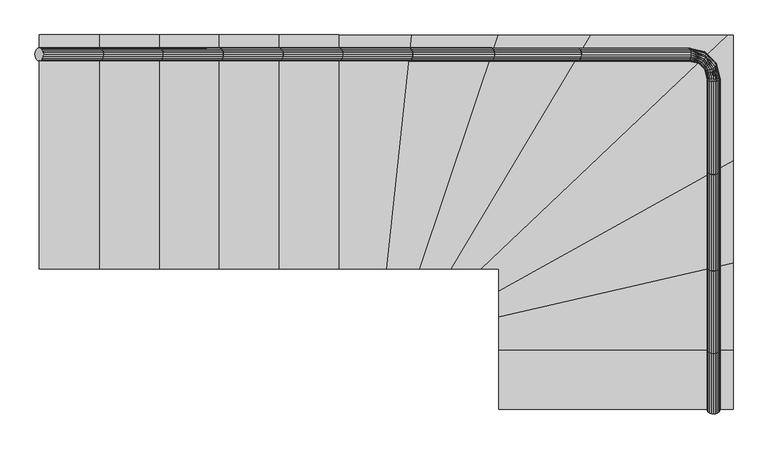
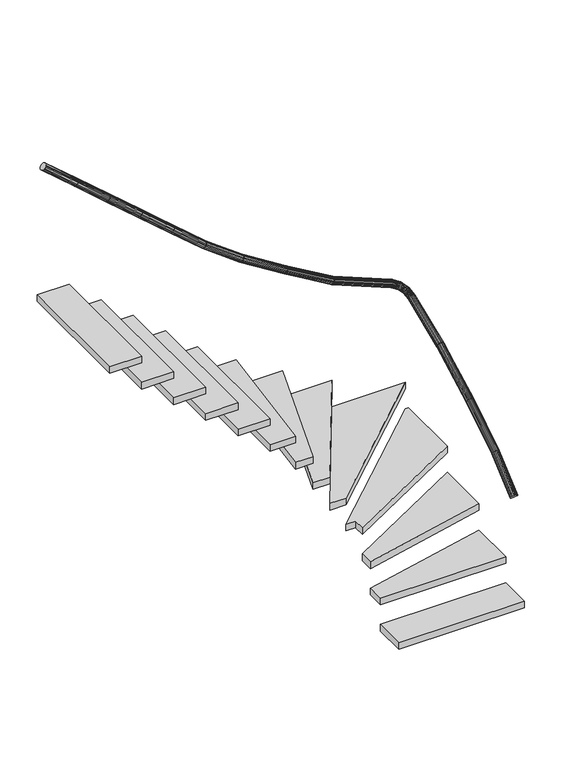
"""IFC4 building model written with IfcOpenShell, lengths in millimetres: stair geometry, 0_3d."""

from ifc_helpers import new_model, si_unit, frame, origin, origin_with_axes, place, context, project, spatial, polyline, outline, extrude, faceted_brep, source, transform, mapped, element, save


def stair_b834b6f4(model_context):
    return source(origin(), model_context, "Body", "SolidModel", [
        faceted_brep([(1747.6382113, 1405.678272, 2054.1646194), (1751.801684, 1406.9018591, 2060.987808), (1755.9651567, 1405.678272, 2067.8109967), (1759.7210797, 1402.127284, 2073.966284), (1762.701797, 1396.5964904, 2078.8511477), (1764.6155354, 1389.627284, 2081.9874233), (1765.2749647, 1381.9018591, 2083.0681102), (1764.6155354, 1374.1764343, 2081.9874233), (1762.701797, 1367.2072278, 2078.8511477), (1759.7210797, 1361.6764343, 2073.966284), (1755.9651567, 1358.1254462, 2067.8109967), (1751.801684, 1356.9018591, 2060.987808), (1747.6382113, 1358.1254462, 2054.1646194), (1743.8822884, 1361.6764343, 2048.009332), (1740.901571, 1367.2072278, 2043.1244683), (1738.9878327, 1374.1764343, 2039.9881928), (1738.3284034, 1381.9018591, 2038.9075058), (1738.9878327, 1389.627284, 2039.9881928), (1740.901571, 1396.5964904, 2043.1244683), (1743.8822884, 1402.127284, 2048.009332), (1441.1651504, 1405.678272, 2266.1670868), (1436.659926, 1406.9018591, 2259.5592366), (1432.1547015, 1405.678272, 2252.9513864), (1428.0904799, 1402.127284, 2246.9903587), (1424.8650953, 1396.5964904, 2242.2596602), (1422.7942709, 1389.627284, 2239.2223649), (1422.0807134, 1381.9018591, 2238.1757842), (1422.7942709, 1374.1764343, 2239.2223649), (1424.8650953, 1367.2072278, 2242.2596602), (1428.0904799, 1361.6764343, 2246.9903587), (1432.1547015, 1358.1254462, 2252.9513864), (1436.659926, 1356.9018591, 2259.5592366), (1441.1651504, 1358.1254462, 2266.1670868), (1445.2293721, 1361.6764343, 2272.1281145), (1448.4547567, 1367.2072278, 2276.858813), (1450.5255811, 1374.1764343, 2279.8961083), (1451.2391385, 1381.9018591, 2280.942689), (1450.5255811, 1389.627284, 2279.8961083), (1448.4547567, 1396.5964904, 2276.858813), (1445.2293721, 1402.127284, 2272.1281145)], [[[0, 1, 2, 3, 4, 5, 6, 7, 8, 9, 10, 11, 12, 13, 14, 15, 16, 17, 18, 19]], [[20, 21, 22, 23, 24, 25, 26, 27, 28, 29, 30, 31, 32, 33, 34, 35, 36, 37, 38, 39]], [[2, 1, 21, 20]], [[3, 2, 20, 39]], [[4, 3, 39, 38]], [[5, 4, 38, 37]], [[6, 5, 37, 36]], [[7, 6, 36, 35]], [[8, 7, 35, 34]], [[9, 8, 34, 33]], [[10, 9, 33, 32]], [[11, 10, 32, 31]], [[12, 11, 31, 30]], [[13, 12, 30, 29]], [[14, 13, 29, 28]], [[15, 14, 28, 27]], [[16, 15, 27, 26]], [[17, 16, 26, 25]], [[18, 17, 25, 24]], [[19, 18, 24, 23]], [[0, 19, 23, 22]], [[1, 0, 22, 21]]]),
        faceted_brep([(2630.2801086, 566.7337566, 1259.7925307), (2631.5036957, 562.7078511, 1266.7020937), (2630.2801086, 558.6819455, 1273.6116568), (2626.7291206, 555.0501237, 1279.8448636), (2621.198327, 552.1678935, 1284.7915646), (2614.2291206, 550.3173878, 1287.9675421), (2606.5036957, 549.679747, 1289.0619094), (2598.7782709, 550.3173878, 1287.9675421), (2591.8090644, 552.1678935, 1284.7915646), (2586.2782709, 555.0501237, 1279.8448636), (2582.7272828, 558.6819455, 1273.6116568), (2581.5036957, 562.7078511, 1266.7020937), (2582.7272828, 566.7337566, 1259.7925307), (2586.2782709, 570.3655785, 1253.5593239), (2591.8090644, 573.2478087, 1248.6126229), (2598.7782709, 575.0983143, 1245.4366454), (2606.5036957, 575.7359551, 1244.3422781), (2614.2291206, 575.0983143, 1245.4366454), (2621.198327, 573.2478087, 1248.6126229), (2626.7291206, 570.3655785, 1253.5593239), (2630.2801086, 928.1440687, 1472.4992177), (2631.5036957, 931.5827131, 1465.2735223), (2630.2801086, 935.0213576, 1458.0478269), (2626.7291206, 938.1234035, 1451.529433), (2621.198327, 940.5852011, 1446.3564062), (2614.2291206, 942.1657724, 1443.0351186), (2606.5036957, 942.7104002, 1441.8906809), (2598.7782709, 942.1657724, 1443.0351186), (2591.8090644, 940.5852011, 1446.3564062), (2586.2782709, 938.1234035, 1451.529433), (2582.7272828, 935.0213576, 1458.0478269), (2581.5036957, 931.5827131, 1465.2735223), (2582.7272828, 928.1440687, 1472.4992177), (2586.2782709, 925.0420228, 1479.0176117), (2591.8090644, 922.5802252, 1484.1906384), (2598.7782709, 920.9996538, 1487.511926), (2606.5036957, 920.4550261, 1488.6563638), (2614.2291206, 920.9996538, 1487.511926), (2621.198327, 922.5802252, 1484.1906384), (2626.7291206, 925.0420228, 1479.0176117)], [[[0, 1, 2, 3, 4, 5, 6, 7, 8, 9, 10, 11, 12, 13, 14, 15, 16, 17, 18, 19]], [[20, 21, 22, 23, 24, 25, 26, 27, 28, 29, 30, 31, 32, 33, 34, 35, 36, 37, 38, 39]], [[2, 1, 21, 20]], [[3, 2, 20, 39]], [[4, 3, 39, 38]], [[5, 4, 38, 37]], [[6, 5, 37, 36]], [[7, 6, 36, 35]], [[8, 7, 35, 34]], [[9, 8, 34, 33]], [[10, 9, 33, 32]], [[11, 10, 32, 31]], [[12, 11, 31, 30]], [[13, 12, 30, 29]], [[14, 13, 29, 28]], [[15, 14, 28, 27]], [[16, 15, 27, 26]], [[17, 16, 26, 25]], [[18, 17, 25, 24]], [[19, 18, 24, 23]], [[0, 19, 23, 22]], [[1, 0, 22, 21]]]),
        extrude(outline(polyline([(1781.5036957, 246.9018591), (1781.5036957, 373.9346688), (2681.5036957, 579.8690495), (2681.5036957, 246.9018591), (1781.5036957, 246.9018591)])), frame((0.0, 0.0, 198.5714286), z_axis=(0.0, 0.0, 1.0), x_axis=(1.0, 0.0, 0.0)), (0.0, 0.0, 1.0), 50.0),
        extrude(outline(polyline([(706.9018591, 556.9018591), (476.9018591, 556.9018591), (476.9018591, 1456.9018591), (706.9018591, 1456.9018591), (706.9018591, 556.9018591)])), frame((0.0, 0.0, 1985.7142857), z_axis=(0.0, 0.0, 1.0), x_axis=(1.0, 0.0, 0.0)), (0.0, 0.0, 1.0), 50.0),
        extrude(outline(polyline([(1781.5036957, 473.824936), (1781.5036957, 556.9018591), (1711.5036957, 556.9018591), (2658.8332796, 1456.9018591), (2681.5036957, 1456.9018591), (2681.5036957, 973.1970565), (1781.5036957, 473.824936)])), frame((0.0, 0.0, 595.7142857), z_axis=(0.0, 0.0, 1.0), x_axis=(1.0, 0.0, 0.0)), (0.0, 0.0, 1.0), 50.0),
        extrude(outline(polyline([(246.9018591, 556.9018591), (16.9018591, 556.9018591), (16.9018591, 1456.9018591), (246.9018591, 1456.9018591), (246.9018591, 556.9018591)])), frame((0.0, 0.0, 2382.8571429), z_axis=(0.0, 0.0, 1.0), x_axis=(1.0, 0.0, 0.0)), (0.0, 0.0, 1.0), 50.0),
        extrude(outline(polyline([(1.2235871, -7.9923214), (0.0, 0.0), (1.2235871, 7.9923214), (4.7745751, 15.2022987), (10.3053687, 20.9241691), (17.2745751, 24.597836), (25.0, 25.8636953), (32.7254248, 24.597836), (39.6946313, 20.9241691), (45.2254248, 15.2022987), (48.7764129, 7.9923214), (50.0, 0.0), (48.7764129, -7.9923214), (45.2254248, -15.2022986), (39.6946313, -20.9241689), (32.7254248, -24.5978359), (25.0, -25.8636953), (17.2745751, -24.5978359), (10.3053687, -20.9241689), (4.7745751, -15.2022986), (1.2235871, -7.9923214)])), frame((936.9018591, 1406.9018591, 2656.7020937), z_axis=(-0.7569287102857389, 0.0, 0.6534974579485127), x_axis=(0.0, -1.0, 0.0)), (0.0, 0.0, 1.0), 303.8595272),
        extrude(outline(polyline([(1.2235871, -7.9923214), (0.0, 0.0), (1.2235871, 7.9923214), (4.7745751, 15.2022986), (10.3053687, 20.9241691), (17.2745751, 24.5978359), (25.0, 25.8636953), (32.7254248, 24.5978359), (39.6946313, 20.9241691), (45.2254248, 15.2022986), (48.7764129, 7.9923214), (50.0, 0.0), (48.7764129, -7.9923214), (45.2254248, -15.2022986), (39.6946313, -20.9241689), (32.7254248, -24.5978359), (25.0, -25.8636953), (17.2745751, -24.5978359), (10.3053687, -20.9241689), (4.7745751, -15.2022986), (1.2235871, -7.9923214)])), frame((706.9018591, 1406.9018591, 2855.2735223), z_axis=(-0.7569287102857376, 0.0, 0.6534974579485142), x_axis=(0.0, -1.0, 0.0)), (0.0, 0.0, 1.0), 303.8595272),
        faceted_brep([(1161.9138744, 1405.678272, 2451.8781793), (1166.9018591, 1406.9018591, 2458.1306652), (1171.8898438, 1405.678272, 2464.383151), (1176.3895699, 1402.127284, 2470.0236), (1179.9605727, 1396.5964904, 2474.4998856), (1182.2532976, 1389.627284, 2477.3738379), (1183.0433167, 1381.9018591, 2478.3641344), (1182.2532976, 1374.1764343, 2477.3738379), (1179.9605727, 1367.2072278, 2474.4998856), (1176.3895699, 1361.6764343, 2470.0236), (1171.8898438, 1358.1254462, 2464.383151), (1166.9018591, 1356.9018591, 2458.1306652), (1161.9138744, 1358.1254462, 2451.8781793), (1157.4141484, 1361.6764343, 2446.2377304), (1153.8431456, 1367.2072278, 2441.7614447), (1151.5504206, 1374.1764343, 2438.8874925), (1150.7604015, 1381.9018591, 2437.897196), (1151.5504206, 1389.627284, 2438.8874925), (1153.8431456, 1396.5964904, 2441.7614447), (1157.4141484, 1402.127284, 2446.2377304), (942.1248208, 1405.678272, 2662.7517113), (936.9018591, 1406.9018591, 2656.7020937), (931.6788974, 1405.678272, 2650.6524762), (926.9671956, 1402.127284, 2645.1950374), (923.2279679, 1396.5964904, 2640.8639895), (920.8272359, 1389.627284, 2638.0832855), (920.0, 1381.9018591, 2637.1251202), (920.8272359, 1374.1764343, 2638.0832855), (923.2279679, 1367.2072278, 2640.8639895), (926.9671956, 1361.6764343, 2645.1950374), (931.6788974, 1358.1254462, 2650.6524762), (936.9018591, 1356.9018591, 2656.7020937), (942.1248208, 1358.1254462, 2662.7517113), (946.8365226, 1361.6764343, 2668.2091501), (950.5757504, 1367.2072278, 2672.540198), (952.9764824, 1374.1764343, 2675.320902), (953.8037182, 1381.9018591, 2676.2790673), (952.9764824, 1389.627284, 2675.320902), (950.5757504, 1396.5964904, 2672.540198), (946.8365226, 1402.127284, 2668.2091501)], [[[0, 1, 2, 3, 4, 5, 6, 7, 8, 9, 10, 11, 12, 13, 14, 15, 16, 17, 18, 19]], [[20, 21, 22, 23, 24, 25, 26, 27, 28, 29, 30, 31, 32, 33, 34, 35, 36, 37, 38, 39]], [[2, 1, 21, 20]], [[3, 2, 20, 39]], [[4, 3, 39, 38]], [[5, 4, 38, 37]], [[6, 5, 37, 36]], [[7, 6, 36, 35]], [[8, 7, 35, 34]], [[9, 8, 34, 33]], [[10, 9, 33, 32]], [[11, 10, 32, 31]], [[12, 11, 31, 30]], [[13, 12, 30, 29]], [[14, 13, 29, 28]], [[15, 14, 28, 27]], [[16, 15, 27, 26]], [[17, 16, 26, 25]], [[18, 17, 25, 24]], [[19, 18, 24, 23]], [[0, 19, 23, 22]], [[1, 0, 22, 21]]]),
        extrude(outline(polyline([(1.2235871, -7.9923214), (0.0, 0.0), (1.2235871, 7.9923214), (4.7745751, 15.2022986), (10.3053687, 20.924169), (17.2745751, 24.5978359), (25.0, 25.8636953), (32.7254248, 24.5978359), (39.6946313, 20.924169), (45.2254248, 15.2022986), (48.7764129, 7.9923214), (50.0, 0.0), (48.7764129, -7.9923214), (45.2254248, -15.2022986), (39.6946313, -20.924169), (32.7254248, -24.597836), (25.0, -25.8636953), (17.2745751, -24.597836), (10.3053687, -20.924169), (4.7745751, -15.2022986), (1.2235871, -7.9923214)])), frame((246.9018591, 1406.9018591, 3252.4163795), z_axis=(-0.7569287102857456, 0.0, 0.6534974579485049), x_axis=(0.0, -1.0, 0.0)), (0.0, 0.0, 1.0), 303.8595272),
        faceted_brep([(2630.2801086, 935.0213576, 1458.0478269), (2631.5036957, 931.5827131, 1465.2735223), (2630.2801086, 928.1440687, 1472.4992177), (2626.7291206, 925.0420228, 1479.0176117), (2621.198327, 922.5802252, 1484.1906384), (2614.2291206, 920.9996538, 1487.511926), (2606.5036957, 920.4550261, 1488.6563638), (2598.7782709, 920.9996538, 1487.511926), (2591.8090644, 922.5802252, 1484.1906384), (2586.2782709, 925.0420228, 1479.0176117), (2582.7272828, 928.1440687, 1472.4992177), (2581.5036957, 931.5827131, 1465.2735223), (2582.7272828, 935.0213576, 1458.0478269), (2586.2782709, 938.1234035, 1451.529433), (2591.8090644, 940.5852011, 1446.3564062), (2598.7782709, 942.1657724, 1443.0351186), (2606.5036957, 942.7104002, 1441.8906809), (2614.2291206, 942.1657724, 1443.0351186), (2621.198327, 940.5852011, 1446.3564062), (2626.7291206, 938.1234035, 1451.529433), (2630.2801086, 1283.3224302, 1620.3777918), (2631.5036957, 1286.3944101, 1612.9994356), (2630.2801086, 1289.46639, 1605.6210794), (2626.7291206, 1292.2376632, 1598.9649681), (2621.198327, 1294.436958, 1593.6826483), (2614.2291206, 1295.8489921, 1590.2911902), (2606.5036957, 1296.335546, 1589.1225734), (2598.7782709, 1295.8489921, 1590.2911902), (2591.8090644, 1294.436958, 1593.6826483), (2586.2782709, 1292.2376632, 1598.9649681), (2582.7272828, 1289.46639, 1605.6210794), (2581.5036957, 1286.3944101, 1612.9994356), (2582.7272828, 1283.3224302, 1620.3777918), (2586.2782709, 1280.5511571, 1627.0339031), (2591.8090644, 1278.3518623, 1632.3162229), (2598.7782709, 1276.9398281, 1635.707681), (2606.5036957, 1276.4532743, 1636.8762979), (2614.2291206, 1276.9398281, 1635.707681), (2621.198327, 1278.3518623, 1632.3162229), (2626.7291206, 1280.5511571, 1627.0339031)], [[[0, 1, 2, 3, 4, 5, 6, 7, 8, 9, 10, 11, 12, 13, 14, 15, 16, 17, 18, 19]], [[20, 21, 22, 23, 24, 25, 26, 27, 28, 29, 30, 31, 32, 33, 34, 35, 36, 37, 38, 39]], [[2, 1, 21, 20]], [[3, 2, 20, 39]], [[4, 3, 39, 38]], [[5, 4, 38, 37]], [[6, 5, 37, 36]], [[7, 6, 36, 35]], [[8, 7, 35, 34]], [[9, 8, 34, 33]], [[10, 9, 33, 32]], [[11, 10, 32, 31]], [[12, 11, 31, 30]], [[13, 12, 30, 29]], [[14, 13, 29, 28]], [[15, 14, 28, 27]], [[16, 15, 27, 26]], [[17, 16, 26, 25]], [[18, 17, 25, 24]], [[19, 18, 24, 23]], [[0, 19, 23, 22]], [[1, 0, 22, 21]]]),
        extrude(outline(polyline([(1.2235871, -7.9923214), (0.0, 0.0), (1.2235871, 7.9923214), (4.7745751, 15.2022986), (10.3053687, 20.9241691), (17.2745751, 24.5978359), (25.0, 25.8636953), (32.7254248, 24.5978359), (39.6946313, 20.9241691), (45.2254248, 15.2022986), (48.7764129, 7.9923214), (50.0, 0.0), (48.7764129, -7.9923214), (45.2254248, -15.2022986), (39.6946313, -20.924169), (32.7254248, -24.5978359), (25.0, -25.8636953), (17.2745751, -24.5978359), (10.3053687, -20.924169), (4.7745751, -15.2022986), (1.2235871, -7.9923214)])), frame((476.9018591, 1406.9018591, 3053.8449509), z_axis=(-0.7569287102857464, 0.0, 0.6534974579485041), x_axis=(0.0, -1.0, 0.0)), (0.0, 0.0, 1.0), 303.8595272),
        faceted_brep([(2630.2801086, 22.1248208, 863.5096191), (2631.5036957, 16.9018591, 869.5592366), (2630.2801086, 11.6788974, 875.6088541), (2626.7291206, 6.9671956, 881.0662929), (2621.198327, 3.2279679, 885.3973409), (2614.2291206, 0.8272359, 888.1780448), (2606.5036957, 0.0, 889.1362101), (2598.7782709, 0.8272359, 888.1780448), (2591.8090644, 3.2279679, 885.3973409), (2586.2782709, 6.9671956, 881.0662929), (2582.7272828, 11.6788974, 875.6088541), (2581.5036957, 16.9018591, 869.5592366), (2582.7272828, 22.1248208, 863.5096191), (2586.2782709, 26.8365226, 858.0521803), (2591.8090644, 30.5757504, 853.7211323), (2598.7782709, 32.9764824, 850.9404284), (2606.5036957, 33.8037182, 849.9822631), (2614.2291206, 32.9764824, 850.9404284), (2621.198327, 30.5757504, 853.7211323), (2626.7291206, 26.8365226, 858.0521803), (2630.2801086, 242.1361647, 1074.5750662), (2631.5036957, 246.9018591, 1068.1306652), (2630.2801086, 251.6675536, 1061.6862641), (2626.7291206, 255.9667486, 1055.872686), (2621.198327, 259.3786091, 1051.2590042), (2614.2291206, 261.5691584, 1048.2968382), (2606.5036957, 262.3239703, 1047.2761453), (2598.7782709, 261.5691584, 1048.2968382), (2591.8090644, 259.3786091, 1051.2590042), (2586.2782709, 255.9667486, 1055.872686), (2582.7272828, 251.6675536, 1061.6862641), (2581.5036957, 246.9018591, 1068.1306652), (2582.7272828, 242.1361647, 1074.5750662), (2586.2782709, 237.8369696, 1080.3886444), (2591.8090644, 234.4251091, 1085.0023262), (2598.7782709, 232.2345598, 1087.9644922), (2606.5036957, 231.4797479, 1088.985185), (2614.2291206, 232.2345598, 1087.9644922), (2621.198327, 234.4251091, 1085.0023262), (2626.7291206, 237.8369696, 1080.3886444)], [[[0, 1, 2, 3, 4, 5, 6, 7, 8, 9, 10, 11, 12, 13, 14, 15, 16, 17, 18, 19]], [[20, 21, 22, 23, 24, 25, 26, 27, 28, 29, 30, 31, 32, 33, 34, 35, 36, 37, 38, 39]], [[2, 1, 21, 20]], [[3, 2, 20, 39]], [[4, 3, 39, 38]], [[5, 4, 38, 37]], [[6, 5, 37, 36]], [[7, 6, 36, 35]], [[8, 7, 35, 34]], [[9, 8, 34, 33]], [[10, 9, 33, 32]], [[11, 10, 32, 31]], [[12, 11, 31, 30]], [[13, 12, 30, 29]], [[14, 13, 29, 28]], [[15, 14, 28, 27]], [[16, 15, 27, 26]], [[17, 16, 26, 25]], [[18, 17, 25, 24]], [[19, 18, 24, 23]], [[0, 19, 23, 22]], [[1, 0, 22, 21]]]),
        extrude(outline(polyline([(1711.5036957, 556.9018591), (1597.1723093, 556.9018591), (2132.6233472, 1456.9018591), (2658.8332796, 1456.9018591), (1711.5036957, 556.9018591)])), frame((0.0, 0.0, 794.2857143), z_axis=(0.0, 0.0, 1.0), x_axis=(1.0, 0.0, 0.0)), (0.0, 0.0, 1.0), 50.0),
        extrude(outline(polyline([(1781.5036957, 16.9018591), (1781.5036957, 246.9018591), (2681.5036957, 246.9018591), (2681.5036957, 16.9018591), (1781.5036957, 16.9018591)])), origin_with_axes(), (0.0, 0.0, 1.0), 50.0),
        extrude(outline(polyline([(1349.1921789, 556.9018591), (1166.9018591, 556.9018591), (1166.9018591, 1456.9018591), (1444.6115394, 1456.9018591), (1349.1921789, 556.9018591)])), frame((0.0, 0.0, 1390.0), z_axis=(0.0, 0.0, 1.0), x_axis=(1.0, 0.0, 0.0)), (0.0, 0.0, 1.0), 50.0),
        extrude(outline(polyline([(1477.0220692, 556.9018591), (1349.1921789, 556.9018591), (1444.6115394, 1456.9018591), (1776.781649, 1456.9018591), (1477.0220692, 556.9018591)])), frame((0.0, 0.0, 1191.4285714), z_axis=(0.0, 0.0, 1.0), x_axis=(1.0, 0.0, 0.0)), (0.0, 0.0, 1.0), 50.0),
        faceted_brep([(1432.1547015, 1405.678272, 2252.9513864), (1436.659926, 1406.9018591, 2259.5592366), (1441.1651504, 1405.678272, 2266.1670868), (1445.2293721, 1402.127284, 2272.1281145), (1448.4547567, 1396.5964904, 2276.858813), (1450.5255811, 1389.627284, 2279.8961083), (1451.2391385, 1381.9018591, 2280.942689), (1450.5255811, 1374.1764343, 2279.8961083), (1448.4547567, 1367.2072278, 2276.858813), (1445.2293721, 1361.6764343, 2272.1281145), (1441.1651504, 1358.1254462, 2266.1670868), (1436.659926, 1356.9018591, 2259.5592366), (1432.1547015, 1358.1254462, 2252.9513864), (1428.0904799, 1361.6764343, 2246.9903587), (1424.8650953, 1367.2072278, 2242.2596602), (1422.7942709, 1374.1764343, 2239.2223649), (1422.0807134, 1381.9018591, 2238.1757842), (1422.7942709, 1389.627284, 2239.2223649), (1424.8650953, 1396.5964904, 2242.2596602), (1428.0904799, 1402.127284, 2246.9903587), (1171.8898438, 1405.678272, 2464.383151), (1166.9018591, 1406.9018591, 2458.1306652), (1161.9138744, 1405.678272, 2451.8781793), (1157.4141484, 1402.127284, 2446.2377304), (1153.8431456, 1396.5964904, 2441.7614447), (1151.5504206, 1389.627284, 2438.8874925), (1150.7604015, 1381.9018591, 2437.897196), (1151.5504206, 1374.1764343, 2438.8874925), (1153.8431456, 1367.2072278, 2441.7614447), (1157.4141484, 1361.6764343, 2446.2377304), (1161.9138744, 1358.1254462, 2451.8781793), (1166.9018591, 1356.9018591, 2458.1306652), (1171.8898438, 1358.1254462, 2464.383151), (1176.3895699, 1361.6764343, 2470.0236), (1179.9605727, 1367.2072278, 2474.4998856), (1182.2532976, 1374.1764343, 2477.3738379), (1183.0433167, 1381.9018591, 2478.3641344), (1182.2532976, 1389.627284, 2477.3738379), (1179.9605727, 1396.5964904, 2474.4998856), (1176.3895699, 1402.127284, 2470.0236)], [[[0, 1, 2, 3, 4, 5, 6, 7, 8, 9, 10, 11, 12, 13, 14, 15, 16, 17, 18, 19]], [[20, 21, 22, 23, 24, 25, 26, 27, 28, 29, 30, 31, 32, 33, 34, 35, 36, 37, 38, 39]], [[2, 1, 21, 20]], [[3, 2, 20, 39]], [[4, 3, 39, 38]], [[5, 4, 38, 37]], [[6, 5, 37, 36]], [[7, 6, 36, 35]], [[8, 7, 35, 34]], [[9, 8, 34, 33]], [[10, 9, 33, 32]], [[11, 10, 32, 31]], [[12, 11, 31, 30]], [[13, 12, 30, 29]], [[14, 13, 29, 28]], [[15, 14, 28, 27]], [[16, 15, 27, 26]], [[17, 16, 26, 25]], [[18, 17, 25, 24]], [[19, 18, 24, 23]], [[0, 19, 23, 22]], [[1, 0, 22, 21]]]),
        extrude(outline(polyline([(936.9018591, 556.9018591), (706.9018591, 556.9018591), (706.9018591, 1456.9018591), (936.9018591, 1456.9018591), (936.9018591, 556.9018591)])), frame((0.0, 0.0, 1787.1428571), z_axis=(0.0, 0.0, 1.0), x_axis=(1.0, 0.0, 0.0)), (0.0, 0.0, 1.0), 50.0),
        faceted_brep([(2630.2801086, 1289.46639, 1605.6210794), (2631.5036957, 1286.3944101, 1612.9994356), (2630.2801086, 1283.3224302, 1620.3777918), (2626.7291206, 1280.5511571, 1627.0339031), (2621.198327, 1278.3518623, 1632.3162229), (2614.2291206, 1276.9398281, 1635.707681), (2606.5036957, 1276.4532743, 1636.8762979), (2598.7782709, 1276.9398281, 1635.707681), (2591.8090644, 1278.3518623, 1632.3162229), (2586.2782709, 1280.5511571, 1627.0339031), (2582.7272828, 1283.3224302, 1620.3777918), (2581.5036957, 1286.3944101, 1612.9994356), (2582.7272828, 1289.46639, 1605.6210794), (2586.2782709, 1292.2376632, 1598.9649681), (2591.8090644, 1294.436958, 1593.6826483), (2598.7782709, 1295.8489921, 1590.2911902), (2606.5036957, 1296.335546, 1589.1225734), (2614.2291206, 1295.8489921, 1590.2911902), (2621.198327, 1294.436958, 1593.6826483), (2626.7291206, 1292.2376632, 1598.9649681), (2616.4980036, 1348.8501513, 1638.9123688), (2617.3046378, 1344.8271855, 1645.879395), (2615.8855438, 1340.0232633, 1652.1644401), (2612.3796323, 1334.9086261, 1657.1522801), (2607.1300863, 1329.9839302, 1660.3546705), (2600.650768, 1325.7312391, 1661.4581391), (2593.5759183, 1322.5668359, 1660.3546705), (2586.5980727, 1320.8004745, 1657.1522801), (2580.4002713, 1320.6050585, 1652.1644401), (2575.5891981, 1321.9997167, 1645.879395), (2572.6357946, 1324.8479302, 1638.9123688), (2571.8291603, 1328.870896, 1631.9453426), (2573.2482544, 1333.6748181, 1625.6602975), (2576.7541659, 1338.7894554, 1620.6724574), (2582.0037118, 1343.7141513, 1617.470067), (2588.4830301, 1347.9668423, 1616.3665985), (2595.5578799, 1351.1312455, 1617.470067), (2602.5357255, 1352.8976069, 1620.6724574), (2608.7335269, 1353.0930229, 1625.6602975), (2613.5446, 1351.6983647, 1631.9453426), (2573.2894856, 1391.9456089, 1666.2859781), (2576.1190741, 1389.0124344, 1673.2691208), (2577.5017941, 1384.2169558, 1679.5687049), (2577.3022952, 1378.028588, 1684.5680831), (2575.5401057, 1371.0530916, 1687.7778814), (2572.3877211, 1363.9732768, 1688.8839026), (2568.1537188, 1357.4821652, 1687.7778814), (2563.2525523, 1352.215152, 1684.5680831), (2558.163982, 1348.6878091, 1679.5687049), (2553.3861126, 1347.2454175, 1673.2691208), (2549.3866353, 1348.0291684, 1666.2859781), (2546.5570467, 1350.962343, 1659.3028354), (2545.1743267, 1355.7578216, 1653.0032514), (2545.3738257, 1361.9461894, 1648.0038732), (2547.1360151, 1368.9216857, 1644.7940748), (2550.2883997, 1376.0015006, 1643.6880537), (2554.5224021, 1382.4926122, 1644.7940748), (2559.4235686, 1387.7596254, 1648.0038732), (2564.5121389, 1391.2869683, 1653.0032514), (2569.2900082, 1392.7293599, 1659.3028354), (2510.6895066, 1406.9018591, 1691.7803901), (2513.6813624, 1405.678272, 1699.1915978), (2516.3803544, 1402.127284, 1705.8773449), (2518.5222867, 1396.5964904, 1711.1831838), (2519.8974918, 1389.627284, 1714.5897421), (2520.3713552, 1381.9018591, 1715.7635621), (2519.8974918, 1374.1764343, 1714.5897421), (2518.5222867, 1367.2072278, 1711.1831838), (2516.3803544, 1361.6764343, 1705.8773449), (2513.6813624, 1358.1254462, 1699.1915978), (2510.6895066, 1356.9018591, 1691.7803901), (2507.6976509, 1358.1254462, 1684.3691823), (2504.9986588, 1361.6764343, 1677.6834352), (2502.8567266, 1367.2072278, 1672.3775963), (2501.4815215, 1374.1764343, 1668.971038), (2501.0076581, 1381.9018591, 1667.797218), (2501.4815215, 1389.627284, 1668.971038), (2502.8567266, 1396.5964904, 1672.3775963), (2504.9986588, 1402.127284, 1677.6834352), (2507.6976509, 1405.678272, 1684.3691823), (2091.5504886, 1405.678272, 1869.6030507), (2088.0024274, 1406.9018591, 1862.4163795), (2084.4543661, 1405.678272, 1855.2297082), (2081.2536138, 1402.127284, 1848.7465184), (2078.7134824, 1396.5964904, 1843.6014299), (2077.0826177, 1389.627284, 1840.2980797), (2076.52066, 1381.9018591, 1839.1598228), (2077.0826177, 1374.1764343, 1840.2980797), (2078.7134824, 1367.2072278, 1843.6014299), (2081.2536138, 1361.6764343, 1848.7465184), (2084.4543661, 1358.1254462, 1855.2297082), (2088.0024274, 1356.9018591, 1862.4163795), (2091.5504886, 1358.1254462, 1869.6030507), (2094.7512409, 1361.6764343, 1876.0862405), (2097.2913723, 1367.2072278, 1881.231329), (2098.9222371, 1374.1764343, 1884.5346792), (2099.4841948, 1381.9018591, 1885.6729361), (2098.9222371, 1389.627284, 1884.5346792), (2097.2913723, 1396.5964904, 1881.231329), (2094.7512409, 1402.127284, 1876.0862405)], [[[0, 1, 2, 3, 4, 5, 6, 7, 8, 9, 10, 11, 12, 13, 14, 15, 16, 17, 18, 19]], [[2, 1, 20]], [[21, 2, 20]], [[3, 2, 21]], [[22, 3, 21]], [[4, 3, 22]], [[23, 4, 22]], [[5, 4, 23]], [[24, 5, 23]], [[6, 5, 24]], [[25, 6, 24]], [[7, 6, 25]], [[26, 7, 25]], [[8, 7, 26]], [[27, 8, 26]], [[9, 8, 27]], [[28, 9, 27]], [[10, 9, 28]], [[29, 10, 28]], [[11, 10, 29]], [[30, 11, 29]], [[12, 11, 30]], [[31, 12, 30]], [[13, 12, 31]], [[32, 13, 31]], [[14, 13, 32]], [[33, 14, 32]], [[15, 14, 33]], [[34, 15, 33]], [[16, 15, 34]], [[35, 16, 34]], [[17, 16, 35]], [[36, 17, 35]], [[18, 17, 36]], [[37, 18, 36]], [[19, 18, 37]], [[38, 19, 37]], [[0, 19, 38]], [[39, 0, 38]], [[1, 0, 39]], [[20, 1, 39]], [[21, 20, 40]], [[41, 21, 40]], [[22, 21, 41]], [[42, 22, 41]], [[23, 22, 42]], [[43, 23, 42]], [[24, 23, 43]], [[44, 24, 43]], [[25, 24, 44]], [[45, 25, 44]], [[26, 25, 45]], [[46, 26, 45]], [[27, 26, 46]], [[47, 27, 46]], [[28, 27, 47]], [[48, 28, 47]], [[29, 28, 48]], [[49, 29, 48]], [[30, 29, 49]], [[50, 30, 49]], [[31, 30, 50]], [[51, 31, 50]], [[32, 31, 51]], [[52, 32, 51]], [[33, 32, 52]], [[53, 33, 52]], [[34, 33, 53]], [[54, 34, 53]], [[35, 34, 54]], [[55, 35, 54]], [[36, 35, 55]], [[56, 36, 55]], [[37, 36, 56]], [[57, 37, 56]], [[38, 37, 57]], [[58, 38, 57]], [[39, 38, 58]], [[59, 39, 58]], [[20, 39, 59]], [[40, 20, 59]], [[41, 40, 60]], [[61, 41, 60]], [[42, 41, 61]], [[62, 42, 61]], [[43, 42, 62]], [[63, 43, 62]], [[44, 43, 63]], [[64, 44, 63]], [[45, 44, 64]], [[65, 45, 64]], [[46, 45, 65]], [[66, 46, 65]], [[47, 46, 66]], [[67, 47, 66]], [[48, 47, 67]], [[68, 48, 67]], [[49, 48, 68]], [[69, 49, 68]], [[50, 49, 69]], [[70, 50, 69]], [[51, 50, 70]], [[71, 51, 70]], [[52, 51, 71]], [[72, 52, 71]], [[53, 52, 72]], [[73, 53, 72]], [[54, 53, 73]], [[74, 54, 73]], [[55, 54, 74]], [[75, 55, 74]], [[56, 55, 75]], [[76, 56, 75]], [[57, 56, 76]], [[77, 57, 76]], [[58, 57, 77]], [[78, 58, 77]], [[59, 58, 78]], [[79, 59, 78]], [[40, 59, 79]], [[60, 40, 79]], [[80, 81, 82, 83, 84, 85, 86, 87, 88, 89, 90, 91, 92, 93, 94, 95, 96, 97, 98, 99]], [[61, 60, 81, 80]], [[62, 61, 80, 99]], [[63, 62, 99, 98]], [[64, 63, 98, 97]], [[65, 64, 97, 96]], [[66, 65, 96, 95]], [[67, 66, 95, 94]], [[68, 67, 94, 93]], [[69, 68, 93, 92]], [[70, 69, 92, 91]], [[71, 70, 91, 90]], [[72, 71, 90, 89]], [[73, 72, 89, 88]], [[74, 73, 88, 87]], [[75, 74, 87, 86]], [[76, 75, 86, 85]], [[77, 76, 85, 84]], [[78, 77, 84, 83]], [[79, 78, 83, 82]], [[60, 79, 82, 81]]]),
        faceted_brep([(2084.4543661, 1405.678272, 1855.2297082), (2088.0024274, 1406.9018591, 1862.4163795), (2091.5504886, 1405.678272, 1869.6030507), (2094.7512409, 1402.127284, 1876.0862405), (2097.2913723, 1396.5964904, 1881.231329), (2098.9222371, 1389.627284, 1884.5346792), (2099.4841948, 1381.9018591, 1885.6729361), (2098.9222371, 1374.1764343, 1884.5346792), (2097.2913723, 1367.2072278, 1881.231329), (2094.7512409, 1361.6764343, 1876.0862405), (2091.5504886, 1358.1254462, 1869.6030507), (2088.0024274, 1356.9018591, 1862.4163795), (2084.4543661, 1358.1254462, 1855.2297082), (2081.2536138, 1361.6764343, 1848.7465184), (2078.7134824, 1367.2072278, 1843.6014299), (2077.0826177, 1374.1764343, 1840.2980797), (2076.52066, 1381.9018591, 1839.1598228), (2077.0826177, 1389.627284, 1840.2980797), (2078.7134824, 1396.5964904, 1843.6014299), (2081.2536138, 1402.127284, 1848.7465184), (1755.9651567, 1405.678272, 2067.8109967), (1751.801684, 1406.9018591, 2060.987808), (1747.6382113, 1405.678272, 2054.1646194), (1743.8822884, 1402.127284, 2048.009332), (1740.901571, 1396.5964904, 2043.1244683), (1738.9878327, 1389.627284, 2039.9881928), (1738.3284034, 1381.9018591, 2038.9075058), (1738.9878327, 1374.1764343, 2039.9881928), (1740.901571, 1367.2072278, 2043.1244683), (1743.8822884, 1361.6764343, 2048.009332), (1747.6382113, 1358.1254462, 2054.1646194), (1751.801684, 1356.9018591, 2060.987808), (1755.9651567, 1358.1254462, 2067.8109967), (1759.7210797, 1361.6764343, 2073.966284), (1762.701797, 1367.2072278, 2078.8511477), (1764.6155354, 1374.1764343, 2081.9874233), (1765.2749647, 1381.9018591, 2083.0681102), (1764.6155354, 1389.627284, 2081.9874233), (1762.701797, 1396.5964904, 2078.8511477), (1759.7210797, 1402.127284, 2073.966284)], [[[0, 1, 2, 3, 4, 5, 6, 7, 8, 9, 10, 11, 12, 13, 14, 15, 16, 17, 18, 19]], [[20, 21, 22, 23, 24, 25, 26, 27, 28, 29, 30, 31, 32, 33, 34, 35, 36, 37, 38, 39]], [[2, 1, 21, 20]], [[3, 2, 20, 39]], [[4, 3, 39, 38]], [[5, 4, 38, 37]], [[6, 5, 37, 36]], [[7, 6, 36, 35]], [[8, 7, 35, 34]], [[9, 8, 34, 33]], [[10, 9, 33, 32]], [[11, 10, 32, 31]], [[12, 11, 31, 30]], [[13, 12, 30, 29]], [[14, 13, 29, 28]], [[15, 14, 28, 27]], [[16, 15, 27, 26]], [[17, 16, 26, 25]], [[18, 17, 25, 24]], [[19, 18, 24, 23]], [[0, 19, 23, 22]], [[1, 0, 22, 21]]]),
        extrude(outline(polyline([(1781.5036957, 373.9346688), (1781.5036957, 473.824936), (2681.5036957, 973.1970565), (2681.5036957, 579.8690495), (1781.5036957, 373.9346688)])), frame((0.0, 0.0, 397.1428571), z_axis=(0.0, 0.0, 1.0), x_axis=(1.0, 0.0, 0.0)), (0.0, 0.0, 1.0), 50.0),
        faceted_brep([(2630.2801086, 251.6675536, 1061.6862641), (2631.5036957, 246.9018591, 1068.1306652), (2630.2801086, 242.1361647, 1074.5750662), (2626.7291206, 237.8369696, 1080.3886444), (2621.198327, 234.4251091, 1085.0023262), (2614.2291206, 232.2345598, 1087.9644922), (2606.5036957, 231.4797479, 1088.985185), (2598.7782709, 232.2345598, 1087.9644922), (2591.8090644, 234.4251091, 1085.0023262), (2586.2782709, 237.8369696, 1080.3886444), (2582.7272828, 242.1361647, 1074.5750662), (2581.5036957, 246.9018591, 1068.1306652), (2582.7272828, 251.6675536, 1061.6862641), (2586.2782709, 255.9667486, 1055.872686), (2591.8090644, 259.3786091, 1051.2590042), (2598.7782709, 261.5691584, 1048.2968382), (2606.5036957, 262.3239703, 1047.2761453), (2614.2291206, 261.5691584, 1048.2968382), (2621.198327, 259.3786091, 1051.2590042), (2626.7291206, 255.9667486, 1055.872686), (2630.2801086, 558.6819455, 1273.6116568), (2631.5036957, 562.7078511, 1266.7020937), (2630.2801086, 566.7337566, 1259.7925307), (2626.7291206, 570.3655785, 1253.5593239), (2621.198327, 573.2478087, 1248.6126229), (2614.2291206, 575.0983143, 1245.4366454), (2606.5036957, 575.7359551, 1244.3422781), (2598.7782709, 575.0983143, 1245.4366454), (2591.8090644, 573.2478087, 1248.6126229), (2586.2782709, 570.3655785, 1253.5593239), (2582.7272828, 566.7337566, 1259.7925307), (2581.5036957, 562.7078511, 1266.7020937), (2582.7272828, 558.6819455, 1273.6116568), (2586.2782709, 555.0501237, 1279.8448636), (2591.8090644, 552.1678935, 1284.7915646), (2598.7782709, 550.3173878, 1287.9675421), (2606.5036957, 549.679747, 1289.0619094), (2614.2291206, 550.3173878, 1287.9675421), (2621.198327, 552.1678935, 1284.7915646), (2626.7291206, 555.0501237, 1279.8448636)], [[[0, 1, 2, 3, 4, 5, 6, 7, 8, 9, 10, 11, 12, 13, 14, 15, 16, 17, 18, 19]], [[20, 21, 22, 23, 24, 25, 26, 27, 28, 29, 30, 31, 32, 33, 34, 35, 36, 37, 38, 39]], [[2, 1, 21, 20]], [[3, 2, 20, 39]], [[4, 3, 39, 38]], [[5, 4, 38, 37]], [[6, 5, 37, 36]], [[7, 6, 36, 35]], [[8, 7, 35, 34]], [[9, 8, 34, 33]], [[10, 9, 33, 32]], [[11, 10, 32, 31]], [[12, 11, 31, 30]], [[13, 12, 30, 29]], [[14, 13, 29, 28]], [[15, 14, 28, 27]], [[16, 15, 27, 26]], [[17, 16, 26, 25]], [[18, 17, 25, 24]], [[19, 18, 24, 23]], [[0, 19, 23, 22]], [[1, 0, 22, 21]]]),
        extrude(outline(polyline([(476.9018591, 556.9018591), (246.9018591, 556.9018591), (246.9018591, 1456.9018591), (476.9018591, 1456.9018591), (476.9018591, 556.9018591)])), frame((0.0, 0.0, 2184.2857143), z_axis=(0.0, 0.0, 1.0), x_axis=(1.0, 0.0, 0.0)), (0.0, 0.0, 1.0), 50.0),
        extrude(outline(polyline([(1597.1723093, 556.9018591), (1477.0220692, 556.9018591), (1776.781649, 1456.9018591), (2132.6233472, 1456.9018591), (1597.1723093, 556.9018591)])), frame((0.0, 0.0, 992.8571429), z_axis=(0.0, 0.0, 1.0), x_axis=(1.0, 0.0, 0.0)), (0.0, 0.0, 1.0), 50.0),
        extrude(outline(polyline([(1166.9018591, 556.9018591), (936.9018591, 556.9018591), (936.9018591, 1456.9018591), (1166.9018591, 1456.9018591), (1166.9018591, 556.9018591)])), frame((0.0, 0.0, 1588.5714286), z_axis=(0.0, 0.0, 1.0), x_axis=(1.0, 0.0, 0.0)), (0.0, 0.0, 1.0), 50.0),
    ])


if __name__ == "__main__":
    model = new_model("IFC4")
    model_context = context("Model", 3, world=origin())
    ifc_project = project(units=[si_unit("LENGTHUNIT", "METRE", prefix="MILLI")], contexts=[model_context])
    site = spatial("IfcSite", under=ifc_project)
    building = spatial("IfcBuilding", under=site)
    placement = place(None, origin())
    stair_shape = stair_b834b6f4(model_context)
    element("IfcStair", 1, ObjectType="0_3d", at=placement, inside=building, context=model_context, shape_type="MappedRepresentation", body=[
        mapped(stair_shape, transform((0.0, 0.0, 0.0), x_axis=(1.0, 0.0, 0.0), y_axis=(0.0, 1.0, 0.0), z_axis=(0.0, 0.0, 1.0))),
    ])
    save(model, "model.ifc")

# Revit data of these elements
# Element 1 (IfcStair, "0_3d")
#   Materials on its faces: "*1", "weiss"
# Materials
#   "*1": class "Unassigned", colour RGB 175 175 175, transparency 0
#   "weiss": class "Unassigned", colour RGB 255 255 255, transparency 0
